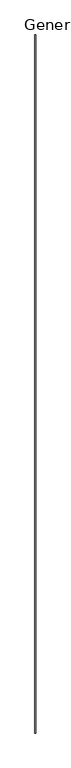
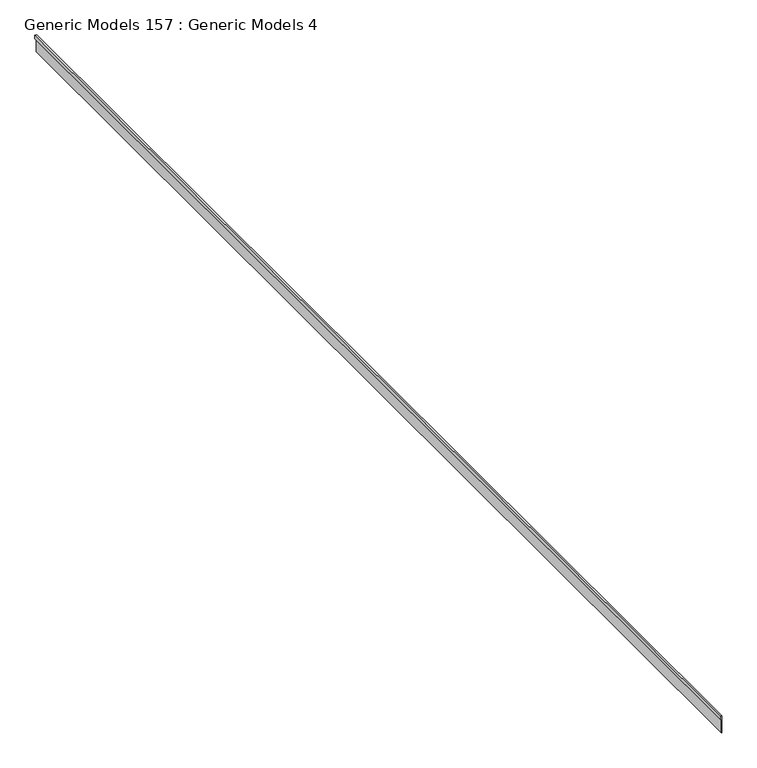
"""IFC4 building model written with IfcOpenShell, lengths in millimetres: proxy geometry, Generic Models 157 : Generic Models 4."""

from ifc_helpers import new_model, si_unit, origin, place, context, project, spatial, faceted_brep, source, transform, mapped, element, save


def generic_models_157_generic_models_4_fb0964b0(model_context):
    return source(origin(), model_context, "Body", "Brep", [
        faceted_brep([(-10236.1097239, -5493.3230338, 122631.7984874), (-10236.1097239, -5493.3230338, 122820.8249647), (-10252.9339552, -5493.3230338, 122820.8249647), (-10252.9339552, -5493.3230338, 122793.7234874), (-10252.9339552, -5493.3230338, 122784.1984874), (-10239.2847239, -5493.3230338, 122784.1984874), (-10239.2847239, -5493.3230338, 122631.7984874), (-10252.9339552, 7054.2769662, 122820.8249648), (-10236.1097239, 7054.2769662, 122820.8249648), (-10236.1097239, 7054.2769662, 122631.7984874), (-10239.2847239, 7054.2769662, 122631.7984874), (-10239.2847239, 7054.2769662, 122784.1984874), (-10252.9339552, 7054.2769662, 122784.1984874), (-10252.9339552, 7054.2769662, 122793.7234874)], [[[0, 1, 2, 3, 4, 5, 6]], [[7, 8, 9, 10, 11, 12, 13]], [[2, 7, 13, 12, 4, 3]], [[9, 0, 6, 10]], [[1, 0, 9, 8]], [[2, 1, 8, 7]], [[5, 11, 10, 6]], [[11, 5, 4, 12]]]),
    ])


if __name__ == "__main__":
    model = new_model("IFC4")
    model_context = context("Model", 3, world=origin())
    ifc_project = project(units=[si_unit("LENGTHUNIT", "METRE", prefix="MILLI")], contexts=[model_context])
    site = spatial("IfcSite", under=ifc_project)
    building = spatial("IfcBuilding", under=site)
    placement = place(None, origin())
    generic_models_157_generic_models_4_shape = generic_models_157_generic_models_4_fb0964b0(model_context)
    element("IfcBuildingElementProxy", 1, Name="Generic Models 157 : Generic Models 4", ObjectType="Generic Models 157 : Generic Models 4", at=placement, inside=building, context=model_context, shape_type="MappedRepresentation", body=[
        mapped(generic_models_157_generic_models_4_shape, transform((0.0, 0.0, 0.0), x_axis=(1.0, 0.0, 0.0), y_axis=(0.0, 1.0, 0.0), z_axis=(0.0, 0.0, 1.0))),
    ])
    save(model, "model.ifc")

# Revit data of these elements
# Element 1 (IfcBuildingElementProxy, "Generic Models 157 : Generic Models 4")
#   Materials on its faces: "_MORTAR SETTING BED"
# Materials
#   "_MORTAR SETTING BED": class "Generic", colour RGB 191 191 191, transparency 0, Cost = 0
